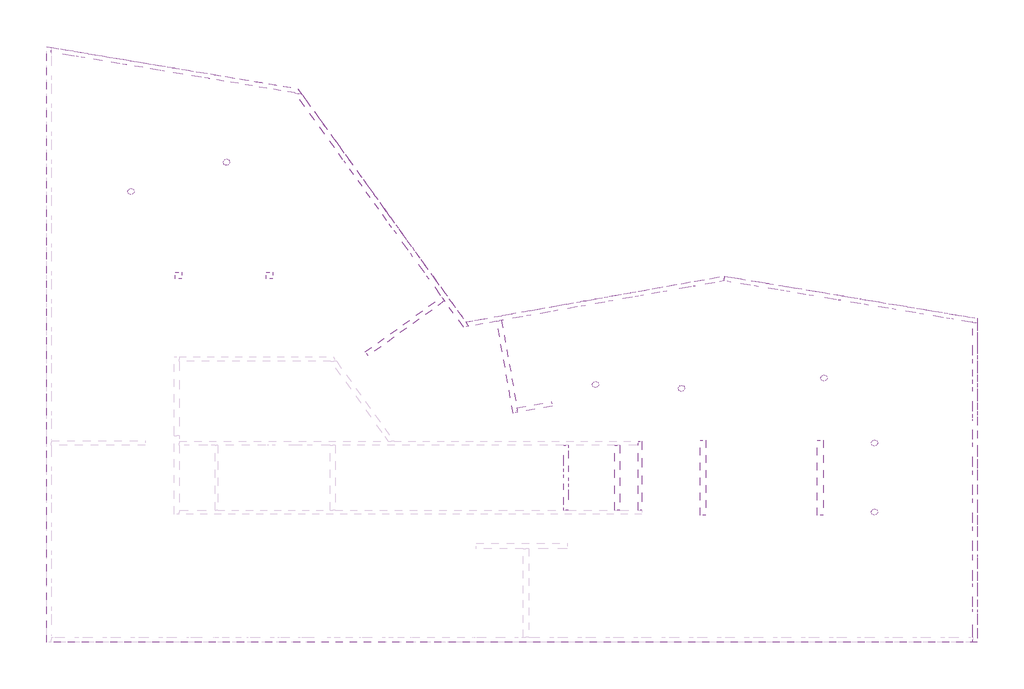
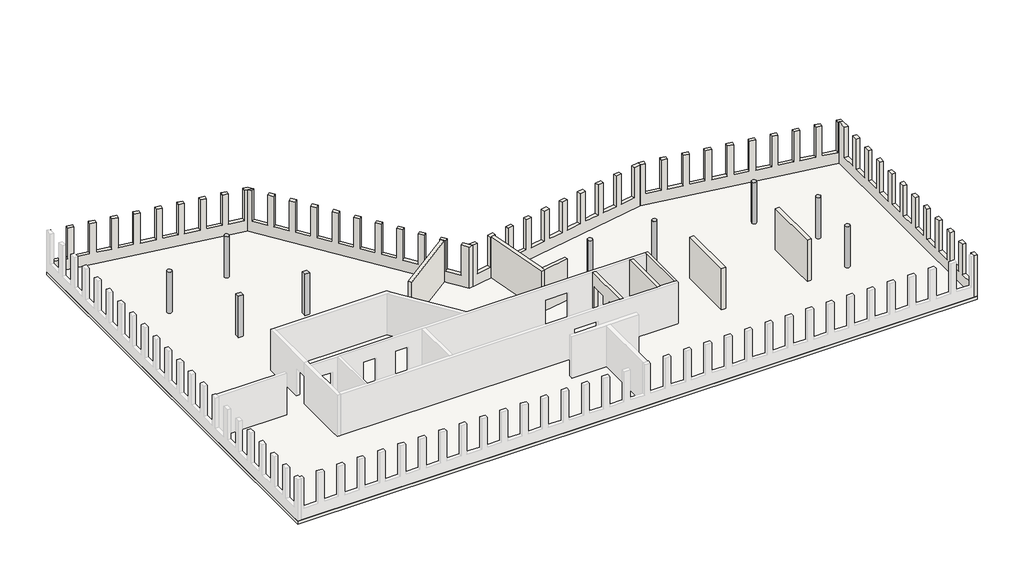
# One storey, part 2 of 2: 13 walls, 9 columns, 1 slab.
"""IFC4 building model written with IfcOpenShell, lengths in millimetres."""

from ifc_helpers import new_model, si_unit, point, frame, frame_2d, origin, place, context, project, spatial, polyline, circle_curve, trimmed, segment, composite_curve, outline, extrude, faceted_brep, element, save

model = new_model("IFC4")

# Units and contexts
model_context = context("Model", 3, world=origin())
ifc_project = project(units=[si_unit("LENGTHUNIT", "METRE", prefix="MILLI")], contexts=[model_context])

# Site, building, storey
site = spatial("IfcSite", under=ifc_project)
building = spatial("IfcBuilding", under=site)
storey = spatial("IfcBuildingStorey", under=building, Name="00_EG_OKFB_0,00", Elevation=0.0)

# Columns
placement = place(None, origin())
element("IfcColumn", 1, ObjectType="5dki STB-Stützen rund : 5dki Stütze rund ø35cm C40/50", at=placement, inside=storey, context=model_context, shape_type="SweptSolid", body=[
    extrude(outline(composite_curve([segment(trimmed(circle_curve(frame_2d((33961.7583834, 13503.0230367)), 175.0), [point((34136.7583834, 13503.0230367))], [point((33786.7583834, 13503.0230367))], False, "CARTESIAN"), True, "CONTINUOUS"), segment(trimmed(circle_curve(frame_2d((33961.7583834, 13503.0230367)), 175.0), [point((33786.7583834, 13503.0230367))], [point((34136.7583834, 13503.0230367))], False, "CARTESIAN"), True, "CONTINUOUS")], self_intersect=False)), frame((0.0, 0.0, 3310.0), z_axis=(0.0, 0.0, 1.0), x_axis=(1.0, 0.0, 0.0)), (0.0, 0.0, 1.0), 3210.0),
])
element("IfcColumn", 2, ObjectType="5dki STB-Stützen rechteckig : 5dki Stütze recht. 35x35cm C35/45", at=placement, inside=storey, context=model_context, shape_type="SweptSolid", body=[
    extrude(outline(polyline([(7139.9999521, 19742.0124565), (7139.9999521, 19392.0124565), (6789.9999521, 19392.0124565), (6789.9999521, 19742.0124565), (7139.9999521, 19742.0124565)])), frame((0.0, 0.0, 3310.0), z_axis=(0.0, 0.0, 1.0), x_axis=(1.0, 0.0, 0.0)), (0.0, 0.0, 1.0), 3210.0),
])
element("IfcColumn", 3, ObjectType="5dki STB-Stützen rechteckig : 5dki Stütze recht. 35x35cm C35/45", at=placement, inside=storey, context=model_context, shape_type="SweptSolid", body=[
    extrude(outline(polyline([(12021.4450432, 19742.0124565), (12021.4450432, 19392.0124565), (11671.4450432, 19392.0124565), (11671.4450432, 19742.0124565), (12021.4450432, 19742.0124565)])), frame((0.0, 0.0, 3310.0), z_axis=(0.0, 0.0, 1.0), x_axis=(1.0, 0.0, 0.0)), (0.0, 0.0, 1.0), 3210.0),
])
element("IfcColumn", 4, ObjectType="5dki STB-Stützen rund : 5dki Stütze rund ø35cm C40/50", at=placement, inside=storey, context=model_context, shape_type="SweptSolid", body=[
    extrude(outline(composite_curve([segment(trimmed(circle_curve(frame_2d((41616.0718251, 14052.9332427)), 175.0), [point((41791.0718251, 14052.9332427))], [point((41441.0718251, 14052.9332427))], False, "CARTESIAN"), True, "CONTINUOUS"), segment(trimmed(circle_curve(frame_2d((41616.0718251, 14052.9332427)), 175.0), [point((41441.0718251, 14052.9332427))], [point((41791.0718251, 14052.9332427))], False, "CARTESIAN"), True, "CONTINUOUS")], self_intersect=False)), frame((0.0, 0.0, 3310.0), z_axis=(0.0, 0.0, 1.0), x_axis=(1.0, 0.0, 0.0)), (0.0, 0.0, 1.0), 3210.0),
])
element("IfcColumn", 5, ObjectType="5dki STB-Stützen rund : 5dki Stütze rund ø35cm C40/50", at=placement, inside=storey, context=model_context, shape_type="SweptSolid", body=[
    extrude(outline(composite_curve([segment(trimmed(circle_curve(frame_2d((44328.9990923, 10566.8309986)), 175.0), [point((44503.9990923, 10566.8309986))], [point((44153.9990923, 10566.8309986))], False, "CARTESIAN"), True, "CONTINUOUS"), segment(trimmed(circle_curve(frame_2d((44328.9990923, 10566.8309986)), 175.0), [point((44153.9990923, 10566.8309986))], [point((44503.9990923, 10566.8309986))], False, "CARTESIAN"), True, "CONTINUOUS")], self_intersect=False)), frame((0.0, 0.0, 3310.0), z_axis=(0.0, 0.0, 1.0), x_axis=(1.0, 0.0, 0.0)), (0.0, 0.0, 1.0), 3210.0),
])
element("IfcColumn", 6, ObjectType="5dki STB-Stützen rund : 5dki Stütze rund ø35cm C40/50", at=placement, inside=storey, context=model_context, shape_type="SweptSolid", body=[
    extrude(outline(composite_curve([segment(trimmed(circle_curve(frame_2d((44328.9990923, 6852.1619165)), 175.0), [point((44503.9990923, 6852.1619165))], [point((44153.9990923, 6852.1619165))], False, "CARTESIAN"), True, "CONTINUOUS"), segment(trimmed(circle_curve(frame_2d((44328.9990923, 6852.1619165)), 175.0), [point((44153.9990923, 6852.1619165))], [point((44503.9990923, 6852.1619165))], False, "CARTESIAN"), True, "CONTINUOUS")], self_intersect=False)), frame((0.0, 0.0, 3310.0), z_axis=(0.0, 0.0, 1.0), x_axis=(1.0, 0.0, 0.0)), (0.0, 0.0, 1.0), 3210.0),
])
element("IfcColumn", 7, ObjectType="5dki STB-Stützen rund : 5dki Stütze rund ø35cm C40/50", at=placement, inside=storey, context=model_context, shape_type="SweptSolid", body=[
    extrude(outline(composite_curve([segment(trimmed(circle_curve(frame_2d((9535.2710874, 25643.9282611)), 175.0), [point((9710.2710874, 25643.9282611))], [point((9360.2710874, 25643.9282611))], False, "CARTESIAN"), True, "CONTINUOUS"), segment(trimmed(circle_curve(frame_2d((9535.2710874, 25643.9282611)), 175.0), [point((9360.2710874, 25643.9282611))], [point((9710.2710874, 25643.9282611))], False, "CARTESIAN"), True, "CONTINUOUS")], self_intersect=False)), frame((0.0, 0.0, 3310.0), z_axis=(0.0, 0.0, 1.0), x_axis=(1.0, 0.0, 0.0)), (0.0, 0.0, 1.0), 3210.0),
])
element("IfcColumn", 8, ObjectType="5dki STB-Stützen rund : 5dki Stütze rund ø35cm C40/50", at=placement, inside=storey, context=model_context, shape_type="SweptSolid", body=[
    extrude(outline(composite_curve([segment(trimmed(circle_curve(frame_2d((4404.9034618, 24066.2757931)), 175.0), [point((4579.9034618, 24066.2757931))], [point((4229.9034618, 24066.2757931))], False, "CARTESIAN"), True, "CONTINUOUS"), segment(trimmed(circle_curve(frame_2d((4404.9034618, 24066.2757931)), 175.0), [point((4229.9034618, 24066.2757931))], [point((4579.9034618, 24066.2757931))], False, "CARTESIAN"), True, "CONTINUOUS")], self_intersect=False)), frame((0.0, 0.0, 3310.0), z_axis=(0.0, 0.0, 1.0), x_axis=(1.0, 0.0, 0.0)), (0.0, 0.0, 1.0), 3210.0),
])
element("IfcColumn", 9, ObjectType="5dki STB-Stützen rund : 5dki Stütze rund ø35cm C40/50", at=placement, inside=storey, context=model_context, shape_type="SweptSolid", body=[
    extrude(outline(composite_curve([segment(trimmed(circle_curve(frame_2d((29357.7423112, 13702.251654)), 175.0), [point((29532.7423112, 13702.251654))], [point((29182.7423112, 13702.251654))], False, "CARTESIAN"), True, "CONTINUOUS"), segment(trimmed(circle_curve(frame_2d((29357.7423112, 13702.251654)), 175.0), [point((29182.7423112, 13702.251654))], [point((29532.7423112, 13702.251654))], False, "CARTESIAN"), True, "CONTINUOUS")], self_intersect=False)), frame((0.0, 0.0, 3310.0), z_axis=(0.0, 0.0, 1.0), x_axis=(1.0, 0.0, 0.0)), (0.0, 0.0, 1.0), 3210.0),
])

# Slab
element("IfcSlab", 10, ObjectType="5dki Decke Ortbeton 25cm C30/37", at=placement, inside=storey, context=model_context, shape_type="SweptSolid", body=[
    extrude(outline(polyline([(-129.9989953, 31855.7150729), (13359.8955383, 29603.0549033), (22383.5041721, 17069.4128529), (36259.9888873, 19532.5499737), (49863.9990833, 17260.8337794), (49863.9991105, -129.9989509), (-129.9989953, -129.9990284), (-129.9989953, 31855.7150729)]), holes=[polyline([(30391.9999891, 10442.0127433), (27891.9999829, 10442.0127433), (27891.9999829, 6960.0000498), (30391.9999891, 6960.0000498), (30391.9999891, 10442.0127433)]), polyline([(31641.9999382, 10442.0127483), (30641.9999891, 10442.0127483), (30641.9999891, 6960.0000514), (31641.9999382, 6960.0000514), (31641.9999382, 10442.0127483)]), polyline([(8916.9999886, 10442.0127052), (6989.9995723, 10442.0127052), (6989.9995723, 6960.0000232), (8916.9999886, 6960.0000232), (8916.9999886, 10442.0127052)]), polyline([(24127.0004657, 8820.0328918), (16927.0004692, 8820.0328918), (16927.0004692, 7020.033352), (24127.0004657, 7020.033352), (24127.0004657, 8820.0328918)])]), frame((0.0, 0.0, 3060.0), z_axis=(0.0, 0.0, 1.0), x_axis=(1.0, 0.0, 0.0)), (0.0, 0.0, 1.0), 250.0),
])

# Walls
element("IfcWall", 11, ObjectType="5dki Lochfassade 26cm C30/37", at=placement, inside=storey, context=model_context, shape_type="Brep", body=[
    faceted_brep([(8967.5024476, 30072.9348316, 4170.0), (8967.5024476, 30072.9348316, 6520.0), (8553.2386546, 30142.1122105, 6520.0), (8553.2386546, 30142.1122105, 4170.0), (7487.988901, 30319.9968993, 4170.0), (7487.988901, 30319.9968993, 6520.0), (7073.7251079, 30389.1742783, 6520.0), (7073.7251079, 30389.1742783, 4170.0), (6008.4753544, 30567.058967, 4170.0), (6008.4753544, 30567.058967, 6520.0), (5594.2115613, 30636.236346, 6520.0), (5594.2115613, 30636.236346, 4170.0), (4528.9618077, 30814.1210348, 4170.0), (4528.9618077, 30814.1210348, 6520.0), (4114.6980147, 30883.2984137, 6520.0), (4114.6980147, 30883.2984137, 4170.0), (3049.4482611, 31061.1831025, 4170.0), (3049.4482611, 31061.1831025, 6520.0), (2635.184468, 31130.3604815, 6520.0), (2635.184468, 31130.3604815, 4170.0), (1569.9347144, 31308.2451702, 4170.0), (1569.9347144, 31308.2451702, 6520.0), (1155.6709214, 31377.4225492, 6520.0), (1155.6709214, 31377.4225492, 4170.0), (130.0010047, 31548.6978518, 4170.0), (130.0010047, 31548.6978518, 3310.0), (13211.4553837, 29364.2425792, 3310.0), (13575.6085618, 29303.4331075, 3310.0), (13575.6085618, 29303.4331075, 6520.0), (13211.4553837, 29364.2425792, 6520.0), (12991.7792945, 29400.9260074, 6520.0), (12991.7792945, 29400.9260074, 4170.0), (11926.5295409, 29578.8106961, 4170.0), (11926.5295409, 29578.8106961, 6520.0), (11512.2657479, 29647.9880751, 6520.0), (11512.2657479, 29647.9880751, 4170.0), (10447.0159943, 29825.8727639, 4170.0), (10447.0159943, 29825.8727639, 6520.0), (10032.7522012, 29895.0501428, 6520.0), (10032.7522012, 29895.0501428, 4170.0), (8596.0627463, 30398.5612253, 6520.0), (9010.3265394, 30329.3838463, 6520.0), (9010.3265394, 30329.3838463, 4170.0), (10075.576293, 30151.4991576, 4170.0), (10075.576293, 30151.4991576, 6520.0), (10489.840086, 30082.3217786, 6520.0), (10489.840086, 30082.3217786, 4170.0), (11555.0898396, 29904.4370898, 4170.0), (11555.0898396, 29904.4370898, 6520.0), (11969.3536327, 29835.2597109, 6520.0), (11969.3536327, 29835.2597109, 4170.0), (13034.6033862, 29657.3750221, 4170.0), (13034.6033862, 29657.3750221, 6520.0), (13359.8955383, 29603.0549033, 6520.0), (13359.8955383, 29603.0549033, 3310.0), (130.0010047, 31812.2980067, 3310.0), (130.0010047, 31812.2980067, 6520.0), (133.2452595, 31811.7562527, 6520.0), (133.2452595, 31811.7562527, 4170.0), (1198.4950131, 31633.8715639, 4170.0), (1198.4950131, 31633.8715639, 6520.0), (1612.7588062, 31564.694185, 6520.0), (1612.7588062, 31564.694185, 4170.0), (2678.0085598, 31386.8094962, 4170.0), (2678.0085598, 31386.8094962, 6520.0), (3092.2723528, 31317.6321172, 6520.0), (3092.2723528, 31317.6321172, 4170.0), (4157.5221064, 31139.7474285, 4170.0), (4157.5221064, 31139.7474285, 6520.0), (4571.7858995, 31070.5700495, 6520.0), (4571.7858995, 31070.5700495, 4170.0), (5637.035653, 30892.6853608, 4170.0), (5637.035653, 30892.6853608, 6520.0), (6051.2994461, 30823.5079818, 6520.0), (6051.2994461, 30823.5079818, 4170.0), (7116.5491997, 30645.623293, 4170.0), (7116.5491997, 30645.623293, 6520.0), (7530.8129927, 30576.4459141, 6520.0), (7530.8129927, 30576.4459141, 4170.0), (8596.0627463, 30398.5612253, 4170.0), (130.0010047, 31792.3282645, 6520.0), (130.0010047, 31792.3282645, 4170.0)], [[[0, 1, 2, 3, 4, 5, 6, 7, 8, 9, 10, 11, 12, 13, 14, 15, 16, 17, 18, 19, 20, 21, 22, 23, 24, 25, 26, 27, 28, 29, 30, 31, 32, 33, 34, 35, 36, 37, 38, 39]], [[40, 41, 42, 43, 44, 45, 46, 47, 48, 49, 50, 51, 52, 53, 54, 55, 56, 57, 58, 59, 60, 61, 62, 63, 64, 65, 66, 67, 68, 69, 70, 71, 72, 73, 74, 75, 76, 77, 78, 79]], [[27, 26, 25, 55, 54]], [[28, 53, 52, 30, 29]], [[48, 34, 33, 49]], [[57, 56, 80]], [[22, 21, 61, 60]], [[18, 17, 65, 64]], [[14, 13, 69, 68]], [[10, 9, 73, 72]], [[6, 5, 77, 76]], [[38, 37, 45, 44]], [[2, 1, 41, 40]], [[56, 55, 25, 24, 81, 80]], [[28, 27, 54, 53]], [[36, 46, 45, 37]], [[47, 35, 34, 48]], [[46, 36, 35, 47]], [[33, 32, 50, 49]], [[31, 30, 52, 51]], [[32, 31, 51, 50]], [[59, 23, 22, 60]], [[81, 58, 57, 80]], [[23, 59, 58, 81, 24]], [[64, 63, 19, 18]], [[62, 61, 21, 20]], [[63, 62, 20, 19]], [[68, 67, 15, 14]], [[66, 65, 17, 16]], [[67, 66, 16, 15]], [[72, 71, 11, 10]], [[70, 69, 13, 12]], [[71, 70, 12, 11]], [[76, 75, 7, 6]], [[74, 73, 9, 8]], [[75, 74, 8, 7]], [[40, 79, 3, 2]], [[78, 77, 5, 4]], [[79, 78, 4, 3]], [[44, 43, 39, 38]], [[42, 41, 1, 0]], [[43, 42, 0, 39]]]),
])
element("IfcWall", 12, ObjectType="5dki Lochfassade 26cm C30/37", at=placement, inside=storey, context=model_context, shape_type="Brep", body=[
    faceted_brep([(22268.004401, 16784.8468851, 6520.0), (21924.4906268, 17261.9817942, 6520.0), (21924.4906268, 17261.9817942, 4170.0), (21293.4697845, 18138.4592307, 4170.0), (21293.4697845, 18138.4592307, 6520.0), (21048.0727903, 18479.3115671, 6520.0), (21048.0727903, 18479.3115671, 4170.0), (20417.0519481, 19355.7890035, 4170.0), (20417.0519481, 19355.7890035, 6520.0), (20171.6549538, 19696.64134, 6520.0), (20171.6549538, 19696.64134, 4170.0), (19540.6341116, 20573.1187764, 4170.0), (19540.6341116, 20573.1187764, 6520.0), (19295.2371174, 20913.9711128, 6520.0), (19295.2371174, 20913.9711128, 4170.0), (18664.2162751, 21790.4485493, 4170.0), (18664.2162751, 21790.4485493, 6520.0), (18418.8192809, 22131.3008857, 6520.0), (18418.8192809, 22131.3008857, 4170.0), (17787.7984387, 23007.7783222, 4170.0), (17787.7984387, 23007.7783222, 6520.0), (17542.4014445, 23348.6306586, 6520.0), (17542.4014445, 23348.6306586, 4170.0), (16911.3806022, 24225.1080951, 4170.0), (16911.3806022, 24225.1080951, 6520.0), (16665.983608, 24565.9604315, 6520.0), (16665.983608, 24565.9604315, 4170.0), (16034.9627658, 25442.4378679, 4170.0), (16034.9627658, 25442.4378679, 6520.0), (15789.5657715, 25783.2902043, 6520.0), (15789.5657715, 25783.2902043, 4170.0), (15158.5449293, 26659.7676408, 4170.0), (15158.5449293, 26659.7676408, 6520.0), (14913.1479351, 27000.6199772, 6520.0), (14913.1479351, 27000.6199772, 4170.0), (14282.1270928, 27877.0974137, 4170.0), (14282.1270928, 27877.0974137, 6520.0), (14036.7300986, 28217.9497501, 6520.0), (14036.7300986, 28217.9497501, 4170.0), (13405.7092564, 29094.4271866, 4170.0), (13405.7092564, 29094.4271866, 6520.0), (13211.4553837, 29364.2425792, 6520.0), (13211.4553837, 29364.2425792, 3310.0), (22268.004401, 16784.8468851, 3310.0), (22135.4944541, 17413.8942192, 4170.0), (22135.4944541, 17413.8942192, 6520.0), (22383.5041721, 17069.4128529, 6520.0), (22552.0750732, 16835.2706799, 6520.0), (22552.0750732, 16835.2706799, 3310.0), (22383.5041721, 17069.4128529, 3310.0), (13575.6085618, 29303.4331075, 3310.0), (13575.6085618, 29303.4331075, 6520.0), (13616.7130837, 29246.3396115, 6520.0), (13616.7130837, 29246.3396115, 4170.0), (14247.7339259, 28369.8621751, 4170.0), (14247.7339259, 28369.8621751, 6520.0), (14493.1309201, 28029.0098387, 6520.0), (14493.1309201, 28029.0098387, 4170.0), (15124.1517624, 27152.5324022, 4170.0), (15124.1517624, 27152.5324022, 6520.0), (15369.5487566, 26811.6800658, 6520.0), (15369.5487566, 26811.6800658, 4170.0), (16000.5695988, 25935.2026293, 4170.0), (16000.5695988, 25935.2026293, 6520.0), (16245.966593, 25594.3502929, 6520.0), (16245.966593, 25594.3502929, 4170.0), (16876.9874353, 24717.8728564, 4170.0), (16876.9874353, 24717.8728564, 6520.0), (17122.3844295, 24377.02052, 6520.0), (17122.3844295, 24377.02052, 4170.0), (17753.4052718, 23500.5430836, 4170.0), (17753.4052718, 23500.5430836, 6520.0), (17998.802266, 23159.6907472, 6520.0), (17998.802266, 23159.6907472, 4170.0), (18629.8231082, 22283.2133107, 4170.0), (18629.8231082, 22283.2133107, 6520.0), (18875.2201024, 21942.3609743, 6520.0), (18875.2201024, 21942.3609743, 4170.0), (19506.2409447, 21065.8835378, 4170.0), (19506.2409447, 21065.8835378, 6520.0), (19751.6379389, 20725.0312014, 6520.0), (19751.6379389, 20725.0312014, 4170.0), (20382.6587811, 19848.5537649, 4170.0), (20382.6587811, 19848.5537649, 6520.0), (20628.0557754, 19507.7014285, 6520.0), (20628.0557754, 19507.7014285, 4170.0), (21259.0766176, 18631.2239921, 4170.0), (21259.0766176, 18631.2239921, 6520.0), (21504.4736118, 18290.3716557, 6520.0), (21504.4736118, 18290.3716557, 4170.0)], [[[0, 1, 2, 3, 4, 5, 6, 7, 8, 9, 10, 11, 12, 13, 14, 15, 16, 17, 18, 19, 20, 21, 22, 23, 24, 25, 26, 27, 28, 29, 30, 31, 32, 33, 34, 35, 36, 37, 38, 39, 40, 41, 42, 43]], [[44, 45, 46, 47, 48, 49, 50, 51, 52, 53, 54, 55, 56, 57, 58, 59, 60, 61, 62, 63, 64, 65, 66, 67, 68, 69, 70, 71, 72, 73, 74, 75, 76, 77, 78, 79, 80, 81, 82, 83, 84, 85, 86, 87, 88, 89]], [[43, 42, 50, 49, 48]], [[51, 41, 40, 52]], [[56, 55, 37, 36]], [[60, 59, 33, 32]], [[64, 63, 29, 28]], [[68, 67, 25, 24]], [[72, 71, 21, 20]], [[76, 75, 17, 16]], [[80, 79, 13, 12]], [[84, 83, 9, 8]], [[88, 87, 5, 4]], [[47, 46, 45, 1, 0]], [[42, 41, 51, 50]], [[0, 43, 48, 47]], [[39, 53, 52, 40]], [[54, 38, 37, 55]], [[53, 39, 38, 54]], [[36, 35, 57, 56]], [[34, 33, 59, 58]], [[35, 34, 58, 57]], [[32, 31, 61, 60]], [[30, 29, 63, 62]], [[31, 30, 62, 61]], [[28, 27, 65, 64]], [[26, 25, 67, 66]], [[27, 26, 66, 65]], [[24, 23, 69, 68]], [[22, 21, 71, 70]], [[23, 22, 70, 69]], [[20, 19, 73, 72]], [[18, 17, 75, 74]], [[19, 18, 74, 73]], [[16, 15, 77, 76]], [[14, 13, 79, 78]], [[15, 14, 78, 77]], [[12, 11, 81, 80]], [[10, 9, 83, 82]], [[11, 10, 82, 81]], [[8, 7, 85, 84]], [[6, 5, 87, 86]], [[7, 6, 86, 85]], [[4, 3, 89, 88]], [[2, 1, 45, 44]], [[3, 2, 44, 89]]]),
])
element("IfcWall", 13, ObjectType="5dki Lochfassade 26cm C30/37", at=placement, inside=storey, context=model_context, shape_type="Brep", body=[
    faceted_brep([(27318.6765704, 17681.3634281, 6520.0), (26924.8330267, 17611.4544654, 6520.0), (26924.8330267, 17611.4544654, 4170.0), (25861.4554587, 17422.7002661, 4170.0), (25861.4554587, 17422.7002661, 6520.0), (25447.9197377, 17349.2958553, 6520.0), (25447.9197377, 17349.2958553, 4170.0), (24384.5421697, 17160.541656, 4170.0), (24384.5421697, 17160.541656, 6520.0), (24300.8505369, 17145.6860228, 6520.0), (24054.698322, 17101.9929211, 6520.0), (23971.0064488, 17087.1372452, 6520.0), (23971.0064488, 17087.1372452, 4170.0), (22907.6288807, 16898.3830459, 4170.0), (22907.6288807, 16898.3830459, 6520.0), (22552.0750732, 16835.2706799, 6520.0), (22552.0750732, 16835.2706799, 3310.0), (24054.698322, 17101.9929211, 3310.0), (24300.8505369, 17145.6860228, 3310.0), (36261.33607, 19268.7248546, 3310.0), (36261.33607, 19268.7248546, 6520.0), (35766.6205834, 19180.910678, 6520.0), (35766.6205834, 19180.910678, 4170.0), (34703.2430153, 18992.1564787, 4170.0), (34703.2430153, 18992.1564787, 6520.0), (34289.7072944, 18918.7520679, 6520.0), (34289.7072944, 18918.7520679, 4170.0), (33226.3297263, 18729.9978686, 4170.0), (33226.3297263, 18729.9978686, 6520.0), (32812.7940054, 18656.5934577, 6520.0), (32812.7940054, 18656.5934577, 4170.0), (31749.4164374, 18467.8392585, 4170.0), (31749.4164374, 18467.8392585, 6520.0), (31335.8807164, 18394.4348476, 6520.0), (31335.8807164, 18394.4348476, 4170.0), (30272.5031484, 18205.6806483, 4170.0), (30272.5031484, 18205.6806483, 6520.0), (29858.9674275, 18132.2762375, 6520.0), (29858.9674275, 18132.2762375, 4170.0), (28795.5898594, 17943.5220382, 4170.0), (28795.5898594, 17943.5220382, 6520.0), (28382.0541385, 17870.1176274, 6520.0), (28382.0541385, 17870.1176274, 4170.0), (27318.6765704, 17681.3634281, 4170.0), (26879.392201, 17867.4527688, 4170.0), (26879.392201, 17867.4527688, 6520.0), (27273.2357447, 17937.3617315, 6520.0), (27273.2357447, 17937.3617315, 4170.0), (28336.6133127, 18126.1159308, 4170.0), (28336.6133127, 18126.1159308, 6520.0), (28750.1490337, 18199.5203416, 6520.0), (28750.1490337, 18199.5203416, 4170.0), (29813.5266017, 18388.2745409, 4170.0), (29813.5266017, 18388.2745409, 6520.0), (30227.0623226, 18461.6789518, 6520.0), (30227.0623226, 18461.6789518, 4170.0), (31290.4398907, 18650.433151, 4170.0), (31290.4398907, 18650.433151, 6520.0), (31703.9756116, 18723.8375619, 6520.0), (31703.9756116, 18723.8375619, 4170.0), (32767.3531797, 18912.5917612, 4170.0), (32767.3531797, 18912.5917612, 6520.0), (33180.8889006, 18985.996172, 6520.0), (33180.8889006, 18985.996172, 4170.0), (34244.2664686, 19174.7503713, 4170.0), (34244.2664686, 19174.7503713, 6520.0), (34657.8021895, 19248.1547821, 6520.0), (34657.8021895, 19248.1547821, 4170.0), (35721.1797576, 19436.9089814, 4170.0), (35721.1797576, 19436.9089814, 6520.0), (36259.9888873, 19532.5499737, 6520.0), (36259.9888873, 19532.5499737, 3310.0), (22383.5041721, 17069.4128529, 3310.0), (22383.5041721, 17069.4128529, 6520.0), (22862.188055, 17154.3813493, 6520.0), (22862.188055, 17154.3813493, 4170.0), (23925.565623, 17343.1355486, 4170.0), (23925.565623, 17343.1355486, 6520.0), (24339.1013439, 17416.5399594, 6520.0), (24339.1013439, 17416.5399594, 4170.0), (25402.478912, 17605.2941587, 4170.0), (25402.478912, 17605.2941587, 6520.0), (25816.0146329, 17678.6985695, 6520.0), (25816.0146329, 17678.6985695, 4170.0)], [[[0, 1, 2, 3, 4, 5, 6, 7, 8, 9, 10, 11, 12, 13, 14, 15, 16, 17, 18, 19, 20, 21, 22, 23, 24, 25, 26, 27, 28, 29, 30, 31, 32, 33, 34, 35, 36, 37, 38, 39, 40, 41, 42, 43]], [[44, 45, 46, 47, 48, 49, 50, 51, 52, 53, 54, 55, 56, 57, 58, 59, 60, 61, 62, 63, 64, 65, 66, 67, 68, 69, 70, 71, 72, 73, 74, 75, 76, 77, 78, 79, 80, 81, 82, 83]], [[19, 18, 17, 16, 72, 71]], [[74, 73, 15, 14]], [[50, 49, 41, 40]], [[37, 36, 54, 53]], [[58, 57, 33, 32]], [[29, 28, 62, 61]], [[21, 20, 70, 69]], [[25, 24, 66, 65]], [[78, 77, 11, 10, 9, 8]], [[82, 81, 5, 4]], [[46, 45, 1, 0]], [[16, 15, 73, 72]], [[20, 19, 71, 70]], [[14, 13, 75, 74]], [[12, 11, 77, 76]], [[13, 12, 76, 75]], [[49, 48, 42, 41]], [[47, 46, 0, 43]], [[48, 47, 43, 42]], [[40, 39, 51, 50]], [[38, 37, 53, 52]], [[39, 38, 52, 51]], [[57, 56, 34, 33]], [[55, 54, 36, 35]], [[56, 55, 35, 34]], [[32, 31, 59, 58]], [[30, 29, 61, 60]], [[31, 30, 60, 59]], [[65, 64, 26, 25]], [[63, 62, 28, 27]], [[64, 63, 27, 26]], [[69, 68, 22, 21]], [[67, 66, 24, 23]], [[68, 67, 23, 22]], [[8, 7, 79, 78]], [[6, 5, 81, 80]], [[7, 6, 80, 79]], [[4, 3, 83, 82]], [[2, 1, 45, 44]], [[3, 2, 44, 83]]]),
])
element("IfcWall", 14, ObjectType="5dki Lochfassade 26cm C30/37", at=placement, inside=storey, context=model_context, shape_type="Brep", body=[
    faceted_brep([(49863.9990837, 16997.2336245, 6520.0), (49603.9990837, 17040.6506907, 6520.0), (49507.8677901, 17056.7035319, 6520.0), (49507.8677901, 17056.7035319, 4170.0), (48442.6180365, 17234.5882205, 4170.0), (48442.6180365, 17234.5882205, 6520.0), (48028.3542434, 17303.7655993, 6520.0), (48028.3542434, 17303.7655993, 4170.0), (46963.1044898, 17481.6502878, 4170.0), (46963.1044898, 17481.6502878, 6520.0), (46548.8406967, 17550.8276667, 6520.0), (46548.8406967, 17550.8276667, 4170.0), (45483.5909431, 17728.7123552, 4170.0), (45483.5909431, 17728.7123552, 6520.0), (45069.32715, 17797.8897341, 6520.0), (45069.32715, 17797.8897341, 4170.0), (44004.0773964, 17975.7744226, 4170.0), (44004.0773964, 17975.7744226, 6520.0), (43589.8136033, 18044.9518015, 6520.0), (43589.8136033, 18044.9518015, 4170.0), (42524.5638497, 18222.83649, 4170.0), (42524.5638497, 18222.83649, 6520.0), (42110.3000566, 18292.0138689, 6520.0), (42110.3000566, 18292.0138689, 4170.0), (41045.050303, 18469.8985574, 4170.0), (41045.050303, 18469.8985574, 6520.0), (40630.7865099, 18539.0759362, 6520.0), (40630.7865099, 18539.0759362, 4170.0), (39565.5367563, 18716.9606248, 4170.0), (39565.5367563, 18716.9606248, 6520.0), (39151.2729632, 18786.1380036, 6520.0), (39151.2729632, 18786.1380036, 4170.0), (38086.0232096, 18964.0226921, 4170.0), (38086.0232096, 18964.0226921, 6520.0), (37671.7594165, 19033.200071, 6520.0), (37671.7594165, 19033.200071, 4170.0), (36606.5096629, 19211.0847595, 4170.0), (36606.5096629, 19211.0847595, 6520.0), (36261.33607, 19268.7248546, 6520.0), (36261.33607, 19268.7248546, 3310.0), (49603.9990837, 17040.6506907, 3310.0), (49863.9990837, 16997.2336245, 3310.0), (49550.6918818, 17313.1525467, 4170.0), (49550.6918818, 17313.1525467, 6520.0), (49863.9990833, 17260.8337794, 6520.0), (49863.9990833, 17260.8337794, 3310.0), (36259.9888873, 19532.5499737, 3310.0), (36259.9888873, 19532.5499737, 6520.0), (36649.3337546, 19467.5337743, 6520.0), (36649.3337546, 19467.5337743, 4170.0), (37714.5835082, 19289.6490858, 4170.0), (37714.5835082, 19289.6490858, 6520.0), (38128.8473013, 19220.4717069, 6520.0), (38128.8473013, 19220.4717069, 4170.0), (39194.0970549, 19042.5870184, 4170.0), (39194.0970549, 19042.5870184, 6520.0), (39608.360848, 18973.4096395, 6520.0), (39608.360848, 18973.4096395, 4170.0), (40673.6106016, 18795.524951, 4170.0), (40673.6106016, 18795.524951, 6520.0), (41087.8743947, 18726.3475721, 6520.0), (41087.8743947, 18726.3475721, 4170.0), (42153.1241483, 18548.4628836, 4170.0), (42153.1241483, 18548.4628836, 6520.0), (42567.3879414, 18479.2855048, 6520.0), (42567.3879414, 18479.2855048, 4170.0), (43632.637695, 18301.4008162, 4170.0), (43632.637695, 18301.4008162, 6520.0), (44046.9014881, 18232.2234374, 6520.0), (44046.9014881, 18232.2234374, 4170.0), (45112.1512417, 18054.3387489, 4170.0), (45112.1512417, 18054.3387489, 6520.0), (45526.4150348, 17985.16137, 6520.0), (45526.4150348, 17985.16137, 4170.0), (46591.6647884, 17807.2766815, 4170.0), (46591.6647884, 17807.2766815, 6520.0), (47005.9285815, 17738.0993026, 6520.0), (47005.9285815, 17738.0993026, 4170.0), (48071.1783351, 17560.2146141, 4170.0), (48071.1783351, 17560.2146141, 6520.0), (48485.4421282, 17491.0372352, 6520.0), (48485.4421282, 17491.0372352, 4170.0)], [[[0, 1, 2, 3, 4, 5, 6, 7, 8, 9, 10, 11, 12, 13, 14, 15, 16, 17, 18, 19, 20, 21, 22, 23, 24, 25, 26, 27, 28, 29, 30, 31, 32, 33, 34, 35, 36, 37, 38, 39, 40, 41]], [[42, 43, 44, 45, 46, 47, 48, 49, 50, 51, 52, 53, 54, 55, 56, 57, 58, 59, 60, 61, 62, 63, 64, 65, 66, 67, 68, 69, 70, 71, 72, 73, 74, 75, 76, 77, 78, 79, 80, 81]], [[41, 40, 39, 46, 45]], [[48, 47, 38, 37]], [[52, 51, 34, 33]], [[56, 55, 30, 29]], [[60, 59, 26, 25]], [[64, 63, 22, 21]], [[68, 67, 18, 17]], [[72, 71, 14, 13]], [[76, 75, 10, 9]], [[80, 79, 6, 5]], [[44, 43, 2, 1, 0]], [[39, 38, 47, 46]], [[0, 41, 45, 44]], [[37, 36, 49, 48]], [[35, 34, 51, 50]], [[36, 35, 50, 49]], [[33, 32, 53, 52]], [[31, 30, 55, 54]], [[32, 31, 54, 53]], [[29, 28, 57, 56]], [[27, 26, 59, 58]], [[28, 27, 58, 57]], [[25, 24, 61, 60]], [[23, 22, 63, 62]], [[24, 23, 62, 61]], [[21, 20, 65, 64]], [[19, 18, 67, 66]], [[20, 19, 66, 65]], [[17, 16, 69, 68]], [[15, 14, 71, 70]], [[16, 15, 70, 69]], [[13, 12, 73, 72]], [[11, 10, 75, 74]], [[12, 11, 74, 73]], [[9, 8, 77, 76]], [[7, 6, 79, 78]], [[8, 7, 78, 77]], [[5, 4, 81, 80]], [[3, 2, 43, 42]], [[4, 3, 42, 81]]]),
])
element("IfcWall", 15, ObjectType="5dki Lochfassade 26cm C30/37", at=placement, inside=storey, context=model_context, shape_type="Brep", body=[
    faceted_brep([(49603.9991105, -129.9989514, 6520.0), (49603.9991101, 130.0010486, 6520.0), (49603.9991099, 277.0124979, 6520.0), (49603.9991099, 277.0124979, 4170.0), (49603.9991082, 1357.0124979, 4170.0), (49603.9991082, 1357.0124979, 6520.0), (49603.9991075, 1777.0124979, 6520.0), (49603.9991075, 1777.0124979, 4170.0), (49603.9991058, 2857.0124979, 4170.0), (49603.9991058, 2857.0124979, 6520.0), (49603.9991052, 3277.0124979, 6520.0), (49603.9991052, 3277.0124979, 4170.0), (49603.9991035, 4357.0124979, 4170.0), (49603.9991035, 4357.0124979, 6520.0), (49603.9991028, 4777.0124979, 6520.0), (49603.9991028, 4777.0124979, 4170.0), (49603.9991011, 5857.0124979, 4170.0), (49603.9991011, 5857.0124979, 6520.0), (49603.9991005, 6277.0124979, 6520.0), (49603.9991005, 6277.0124979, 4170.0), (49603.9990988, 7357.0124979, 4170.0), (49603.9990988, 7357.0124979, 6520.0), (49603.9990981, 7777.0124979, 6520.0), (49603.9990981, 7777.0124979, 4170.0), (49603.9990964, 8857.0124979, 4170.0), (49603.9990964, 8857.0124979, 6520.0), (49603.9990958, 9277.0124979, 6520.0), (49603.9990958, 9277.0124979, 4170.0), (49603.9990941, 10357.0124979, 4170.0), (49603.9990941, 10357.0124979, 6520.0), (49603.9990934, 10777.0124979, 6520.0), (49603.9990934, 10777.0124979, 4170.0), (49603.9990918, 11857.0124979, 4170.0), (49603.9990918, 11857.0124979, 6520.0), (49603.9990911, 12277.0124979, 6520.0), (49603.9990911, 12277.0124979, 4170.0), (49603.9990894, 13357.0124979, 4170.0), (49603.9990894, 13357.0124979, 6520.0), (49603.9990888, 13777.0124979, 6520.0), (49603.9990888, 13777.0124979, 4170.0), (49603.9990871, 14857.0124979, 4170.0), (49603.9990871, 14857.0124979, 6520.0), (49603.9990864, 15277.0124979, 6520.0), (49603.9990864, 15277.0124979, 4170.0), (49603.9990847, 16357.0124979, 4170.0), (49603.9990847, 16357.0124979, 6520.0), (49603.9990837, 17040.6506907, 6520.0), (49603.9990837, 17040.6506907, 3310.0), (49603.9991101, 130.0010486, 3310.0), (49603.9991105, -129.9989514, 3310.0), (49863.9991099, 277.0124983, 4170.0), (49863.9991099, 277.0124983, 6520.0), (49863.9991105, -129.9989509, 6520.0), (49863.9991105, -129.9989509, 3310.0), (49863.9990837, 16997.2336245, 3310.0), (49863.9990837, 16997.2336245, 6520.0), (49863.9990847, 16357.0124983, 6520.0), (49863.9990847, 16357.0124983, 4170.0), (49863.9990864, 15277.0124983, 4170.0), (49863.9990864, 15277.0124983, 6520.0), (49863.9990871, 14857.0124983, 6520.0), (49863.9990871, 14857.0124983, 4170.0), (49863.9990888, 13777.0124983, 4170.0), (49863.9990888, 13777.0124983, 6520.0), (49863.9990894, 13357.0124983, 6520.0), (49863.9990894, 13357.0124983, 4170.0), (49863.9990911, 12277.0124983, 4170.0), (49863.9990911, 12277.0124983, 6520.0), (49863.9990918, 11857.0124983, 6520.0), (49863.9990918, 11857.0124983, 4170.0), (49863.9990934, 10777.0124983, 4170.0), (49863.9990934, 10777.0124983, 6520.0), (49863.9990941, 10357.0124983, 6520.0), (49863.9990941, 10357.0124983, 4170.0), (49863.9990958, 9277.0124983, 4170.0), (49863.9990958, 9277.0124983, 6520.0), (49863.9990964, 8857.0124983, 6520.0), (49863.9990964, 8857.0124983, 4170.0), (49863.9990981, 7777.0124983, 4170.0), (49863.9990981, 7777.0124983, 6520.0), (49863.9990988, 7357.0124983, 6520.0), (49863.9990988, 7357.0124983, 4170.0), (49863.9991005, 6277.0124983, 4170.0), (49863.9991005, 6277.0124983, 6520.0), (49863.9991011, 5857.0124983, 6520.0), (49863.9991011, 5857.0124983, 4170.0), (49863.9991028, 4777.0124983, 4170.0), (49863.9991028, 4777.0124983, 6520.0), (49863.9991035, 4357.0124983, 6520.0), (49863.9991035, 4357.0124983, 4170.0), (49863.9991052, 3277.0124983, 4170.0), (49863.9991052, 3277.0124983, 6520.0), (49863.9991058, 2857.0124983, 6520.0), (49863.9991058, 2857.0124983, 4170.0), (49863.9991075, 1777.0124983, 4170.0), (49863.9991075, 1777.0124983, 6520.0), (49863.9991082, 1357.0124983, 6520.0), (49863.9991082, 1357.0124983, 4170.0)], [[[0, 1, 2, 3, 4, 5, 6, 7, 8, 9, 10, 11, 12, 13, 14, 15, 16, 17, 18, 19, 20, 21, 22, 23, 24, 25, 26, 27, 28, 29, 30, 31, 32, 33, 34, 35, 36, 37, 38, 39, 40, 41, 42, 43, 44, 45, 46, 47, 48, 49]], [[50, 51, 52, 53, 54, 55, 56, 57, 58, 59, 60, 61, 62, 63, 64, 65, 66, 67, 68, 69, 70, 71, 72, 73, 74, 75, 76, 77, 78, 79, 80, 81, 82, 83, 84, 85, 86, 87, 88, 89, 90, 91, 92, 93, 94, 95, 96, 97]], [[49, 48, 47, 54, 53]], [[55, 46, 45, 56]], [[42, 41, 60, 59]], [[38, 37, 64, 63]], [[34, 33, 68, 67]], [[30, 29, 72, 71]], [[26, 25, 76, 75]], [[22, 21, 80, 79]], [[18, 17, 84, 83]], [[14, 13, 88, 87]], [[10, 9, 92, 91]], [[96, 95, 6, 5]], [[52, 51, 2, 1, 0]], [[47, 46, 55, 54]], [[0, 49, 53, 52]], [[58, 43, 42, 59]], [[44, 57, 56, 45]], [[43, 58, 57, 44]], [[63, 62, 39, 38]], [[61, 60, 41, 40]], [[62, 61, 40, 39]], [[67, 66, 35, 34]], [[65, 64, 37, 36]], [[66, 65, 36, 35]], [[71, 70, 31, 30]], [[69, 68, 33, 32]], [[70, 69, 32, 31]], [[75, 74, 27, 26]], [[73, 72, 29, 28]], [[74, 73, 28, 27]], [[79, 78, 23, 22]], [[77, 76, 25, 24]], [[78, 77, 24, 23]], [[83, 82, 19, 18]], [[81, 80, 21, 20]], [[82, 81, 20, 19]], [[87, 86, 15, 14]], [[85, 84, 17, 16]], [[86, 85, 16, 15]], [[91, 90, 11, 10]], [[89, 88, 13, 12]], [[90, 89, 12, 11]], [[95, 94, 7, 6]], [[93, 92, 9, 8]], [[94, 93, 8, 7]], [[5, 4, 97, 96]], [[3, 2, 51, 50]], [[4, 3, 50, 97]]]),
])
element("IfcWall", 16, ObjectType="5dki STB-Wand Kern 25cm C30/37", at=placement, inside=storey, context=model_context, shape_type="SweptSolid", body=[
    extrude(outline(polyline([(30641.9999891, 10442.0127483), (30641.9999891, 6960.0000501), (30391.9999891, 6960.0000498), (30391.9999891, 10442.0127479), (30641.9999891, 10442.0127483)])), frame((0.0, 0.0, 3310.0), z_axis=(0.0, 0.0, 1.0), x_axis=(1.0, 0.0, 0.0)), (0.0, 0.0, 1.0), 3210.0),
])
element("IfcWall", 17, ObjectType="5dki STB-Wand Kern 25cm C30/37", at=placement, inside=storey, context=model_context, shape_type="SweptSolid", body=[
    extrude(outline(polyline([(3482.0126944, -3210.0), (-2.1e-06, -3210.0), (-2.1e-06, 0.0), (279.9681323, 0.0), (279.9681323, -2260.0), (1414.9681323, -2260.0), (1414.9681323, 0.0), (2067.1995869, 0.0), (2067.1995869, -2260.0), (3202.1995869, -2260.0), (3202.1995869, 0.0), (3482.0126944, 0.0), (3482.0126944, -3210.0)])), frame((27641.9999829, 10442.0127408, 3310.0), z_axis=(1.0, 1.6300916066412081e-09, 0.0), x_axis=(1.6300916066412081e-09, -1.0, 0.0)), (0.0, 0.0, 1.0), 250.0),
])
element("IfcWall", 18, ObjectType="5dki STB-Wand Kern 20cm C35/45", at=placement, inside=storey, context=model_context, shape_type="Brep", body=[
    faceted_brep([(31641.9999912, 10662.0127502, 3310.0), (31641.9999881, 10442.0127502, 3310.0), (31641.9999382, 6960.0000514, 3310.0), (31641.9999382, 6960.0000514, 6520.0), (31641.9999881, 10442.0127502, 6520.0), (31641.9999912, 10662.0127502, 6520.0), (31841.9999912, 10662.0127505, 3310.0), (31841.9999912, 10662.0127505, 6520.0), (31841.9999382, 6960.0000516, 6520.0), (31841.9999382, 6960.0000516, 3310.0)], [[[0, 1, 2, 3, 4, 5]], [[6, 7, 8, 9]], [[2, 1, 0, 6, 9]], [[5, 4, 3, 8, 7]], [[0, 5, 7, 6]], [[3, 2, 9, 8]]]),
])
element("IfcWall", 19, ObjectType="5dki STB-Wand 25cm C30/37", at=placement, inside=storey, context=model_context, shape_type="SweptSolid", body=[
    extrude(outline(polyline([(16994.6178661, 15452.6713643), (21084.845921, 18397.4352698), (21230.9155592, 18194.5469734), (17140.6875043, 15249.783068), (16994.6178661, 15452.6713643)])), frame((0.0, 0.0, 3310.0), z_axis=(0.0, 0.0, 1.0), x_axis=(1.0, 0.0, 0.0)), (0.0, 0.0, 1.0), 3210.0),
])
element("IfcWall", 20, ObjectType="5dki STB-Wand 25cm C30/37", at=placement, inside=storey, context=model_context, shape_type="Brep", body=[
    faceted_brep([(24054.698322, 17101.9929211, 3310.0), (24930.952116, 12165.4742089, 3310.0), (24930.952116, 12165.4742089, 6520.0), (24054.698322, 17101.9929211, 6520.0), (24300.8505369, 17145.6860228, 3310.0), (24300.8505369, 17145.6860228, 6520.0), (25133.4112296, 12455.3195251, 6520.0), (25177.1043309, 12209.1673103, 6520.0), (25177.1043309, 12209.1673103, 3310.0), (25133.4112296, 12455.3195251, 3310.0)], [[[0, 1, 2, 3]], [[4, 5, 6, 7, 8, 9]], [[1, 0, 4, 9, 8]], [[3, 2, 7, 6, 5]], [[0, 3, 5, 4]], [[2, 1, 8, 7]]]),
])
element("IfcWall", 21, ObjectType="5dki STB-Wand 25cm C30/37", at=placement, inside=storey, context=model_context, shape_type="SweptSolid", body=[
    extrude(outline(polyline([(27026.4023238, 12537.4258416), (25177.1043309, 12209.1673103), (25133.4112296, 12455.3195251), (26982.7092225, 12783.5780565), (27026.4023238, 12537.4258416)])), frame((0.0, 0.0, 3310.0), z_axis=(0.0, 0.0, 1.0), x_axis=(1.0, 0.0, 0.0)), (0.0, 0.0, 1.0), 3210.0),
])
element("IfcWall", 22, ObjectType="5dki STB-Wand 30cm C30/37", at=placement, inside=storey, context=model_context, shape_type="SweptSolid", body=[
    extrude(outline(polyline([(34969.9990839, 6680.0000532), (34969.9990776, 10702.0125181), (35269.9990776, 10702.0125186), (35269.9990839, 6680.0000537), (34969.9990839, 6680.0000532)])), frame((0.0, 0.0, 3310.0), z_axis=(0.0, 0.0, 1.0), x_axis=(1.0, 0.0, 0.0)), (0.0, 0.0, 1.0), 3210.0),
])
element("IfcWall", 23, ObjectType="5dki STB-Wand 30cm C30/37", at=placement, inside=storey, context=model_context, shape_type="SweptSolid", body=[
    extrude(outline(polyline([(41269.9990703, 6680.000074), (41269.9990703, 10722.0122605), (41569.9990703, 10722.0122605), (41569.9990703, 6680.000074), (41269.9990703, 6680.000074)])), frame((0.0, 0.0, 3310.0), z_axis=(0.0, 0.0, 1.0), x_axis=(1.0, 0.0, 0.0)), (0.0, 0.0, 1.0), 3210.0),
])

save(model, "model.ifc")

# Revit data of these elements
# Type "5dki STB-Stützen rund : 5dki Stütze rund ø35cm C40/50"
#   cpiFitMatchKey = "5D-KI-STB-OB-ST-RUN"
#   cpiComponentType = "Column"
#   5d Materialgüte = "C40/50"
#   Radius = 0.175 m
#   Durchmesser = 0.350 m
#   5dki Bewehrung Stab kg pro m3 = 0
#   5dki Sichtbeton SB3/SB4 [instance default] = no
#   Structural Material = 5d Beton - Stahlbeton
#   Assembly Code = ""
# Type "5dki STB-Stützen rechteckig : 5dki Stütze recht. 35x35cm C35/45"
#   cpiFitMatchKey = "5D-KI-STB-OB-ST-REC"
#   cpiComponentType = "Column"
#   5d Materialgüte = "C35/45"
#   Tiefe = 0.350 m
#   Breite = 0.350 m
#   5dki Bewehrung Stab kg pro m3 = 0
#   5dki Sichtbeton SB3/SB4 [instance default] = no
#   Structural Material = 5d Beton - Stahlbeton
#   Assembly Code = ""
# Type "5dki Decke Ortbeton 25cm C30/37"
#   cpiComponentType = "Slab"
#   cpiFitMatchKey = "5D-KI-STB-OB-DE"
#   5d Materialgüte = "C30/37"
#   Function = 0
#   5dki WU = no
#   Layers, outside or top first: 0.250 m "5d Beton - Stahlbeton" (function 1)
# Type "5dki Lochfassade 26cm C30/37"
#   Type Comments = ""
#   Description = ""
#   cpiComponentType = "Wall"
#   cpiFitMatchKey = "5D-KI-STB-OB-W-LF"
#   5d Materialgüte = "C35/45"
#   Filter Tragend / Nichttragend = yes
#   5dki WU = no
#   Layers, outside or top first: 0.260 m "5d Beton - Stahlbeton" (function 1)
# Type "5dki STB-Wand Kern 25cm C30/37"
#   Type Comments = ""
#   Description = ""
#   cpiComponentType = "Wall"
#   cpiFitMatchKey = "5D-KI-STB-OB-W-K"
#   5d Materialgüte = "C30/37"
#   Filter Tragend / Nichttragend = yes
#   5dki WU = no
#   Layers, outside or top first: 0.250 m "5d Beton - Stahlbeton" (function 1)
# Type "5dki STB-Wand Kern 20cm C35/45"
#   Type Comments = ""
#   Description = ""
#   cpiComponentType = "Wall"
#   cpiFitMatchKey = "5D-KI-STB-OB-W-K"
#   5d Materialgüte = "C35/45"
#   Filter Tragend / Nichttragend = yes
#   5dki WU = no
#   Layers, outside or top first: 0.200 m "5d Beton - Stahlbeton" (function 1)
# Type "5dki STB-Wand 25cm C30/37"
#   Type Comments = ""
#   Description = ""
#   cpiComponentType = "Wall"
#   cpiFitMatchKey = "5D-KI-STB-OB-W"
#   5d Materialgüte = "C30/37"
#   Filter Tragend / Nichttragend = yes
#   5dki WU = no
#   Layers, outside or top first: 0.250 m "5d Beton - Stahlbeton" (function 1)
# Type "5dki STB-Wand 30cm C30/37"
#   Type Comments = ""
#   Description = ""
#   cpiComponentType = "Wall"
#   cpiFitMatchKey = "5D-KI-STB-OB-W"
#   5d Materialgüte = "C30/37"
#   Filter Tragend / Nichttragend = yes
#   5dki WU = no
#   Layers, outside or top first: 0.300 m "5d Beton - Stahlbeton" (function 1)
# Elements 1, 9 (IfcColumn, "5dki STB-Stützen rund : 5dki Stütze rund ø35cm C40/50")
#   Comments = ""
#   000_080_030_Geschoß = "01_OG"
#   5dki Sichtbeton SB3/SB4 = no
#   Phase Created = Neu
#   Materials on its faces: "5d Beton - Stahlbeton"
# Element 2 (IfcColumn, "5dki STB-Stützen rechteckig : 5dki Stütze recht. 35x35cm C35/45")
#   Comments = ""
#   000_080_030_Geschoß = "01_OG"
#   5dki Sichtbeton SB3/SB4 = no
#   Phase Created = Neu
#   Materials on its faces: "5d Beton - Stahlbeton"
# Element 3 (IfcColumn, "5dki STB-Stützen rechteckig : 5dki Stütze recht. 35x35cm C35/45")
#   000_080_030_Geschoß = "01_OG"
#   5dki Sichtbeton SB3/SB4 = no
#   Phase Created = Neu
#   Materials on its faces: "5d Beton - Stahlbeton"
# Elements 4, 5, 6, 7, 8 (IfcColumn, "5dki STB-Stützen rund : 5dki Stütze rund ø35cm C40/50")
#   000_080_030_Geschoß = "01_OG"
#   5dki Sichtbeton SB3/SB4 = no
#   Phase Created = Neu
#   Materials on its faces: "5d Beton - Stahlbeton"
# Element 10 (IfcSlab, "5dki Decke Ortbeton 25cm C30/37")
#   000_080_030_Geschoß = "00_EG"
#   built-in parameter 1001955 = 2.97613 (stored number, unit not read)
#   Height Offset From Level = 0.000 m
#   built-in parameter 1001954 = 1
#   Phase Created = Neu
#   Materials on its faces: "5d Beton - Stahlbeton"
# Elements 11, 12, 13, 14, 15 (IfcWall, "5dki Lochfassade 26cm C30/37")
#   Comments = ""
#   000_080_030_Geschoß = "01_OG"
#   Top Offset = 0.000 m
#   Base Offset = 0.000 m
#   wall height = 3.210 m
#   Phase Created = Neu
#   Base Constraint = 00_EG_OKRD_3,31
#   Top Constraint = 01_OG_UKRD_6,52
#   Materials on its faces: "5d Beton - Stahlbeton"
# Elements 16, 17 (IfcWall, "5dki STB-Wand Kern 25cm C30/37")
#   Comments = ""
#   000_080_030_Geschoß = "01_OG"
#   Top Offset = 0.000 m
#   Base Offset = 0.000 m
#   wall height = 3.210 m
#   Phase Created = Neu
#   Base Constraint = 00_EG_OKRD_3,31
#   Top Constraint = 01_OG_UKRD_6,52
#   Materials on its faces: "5d Beton - Stahlbeton"
# Element 18 (IfcWall, "5dki STB-Wand Kern 20cm C35/45")
#   Comments = ""
#   000_080_030_Geschoß = "01_OG"
#   Top Offset = 0.000 m
#   Base Offset = 0.000 m
#   wall height = 3.210 m
#   Phase Created = Neu
#   Base Constraint = 00_EG_OKRD_3,31
#   Top Constraint = 01_OG_UKRD_6,52
#   Materials on its faces: "5d Beton - Stahlbeton"
# Elements 19, 20 (IfcWall, "5dki STB-Wand 25cm C30/37")
#   Comments = ""
#   000_080_030_Geschoß = "01_OG"
#   Top Offset = 0.000 m
#   Base Offset = 0.000 m
#   wall height = 3.210 m
#   Phase Created = Neu
#   Base Constraint = 00_EG_OKRD_3,31
#   Top Constraint = 01_OG_UKRD_6,52
#   Materials on its faces: "5d Beton - Stahlbeton"
# Element 21 (IfcWall, "5dki STB-Wand 25cm C30/37")
#   000_080_030_Geschoß = "01_OG"
#   Top Offset = 0.000 m
#   Base Offset = 0.000 m
#   wall height = 3.210 m
#   Phase Created = Neu
#   Base Constraint = 00_EG_OKRD_3,31
#   Top Constraint = 01_OG_UKRD_6,52
#   Materials on its faces: "5d Beton - Stahlbeton"
# Element 22 (IfcWall, "5dki STB-Wand 30cm C30/37")
#   000_080_030_Geschoß = "01_OG"
#   Top Offset = 0.000 m
#   Base Offset = 0.000 m
#   wall height = 3.210 m
#   Phase Created = Neu
#   Base Constraint = 00_EG_OKRD_3,31
#   Top Constraint = 01_OG_UKRD_6,52
#   Materials on its faces: "5d Beton - Stahlbeton"
# Element 23 (IfcWall, "5dki STB-Wand 30cm C30/37")
#   Comments = ""
#   000_080_030_Geschoß = "01_OG"
#   Top Offset = 0.000 m
#   Base Offset = 0.000 m
#   wall height = 3.210 m
#   Phase Created = Neu
#   Base Constraint = 00_EG_OKRD_3,31
#   Top Constraint = 01_OG_UKRD_6,52
#   Materials on its faces: "5d Beton - Stahlbeton"
# Materials
#   "5d Beton - Stahlbeton": class "5dki", colour RGB 200 200 200, transparency 0, Cost = 0
